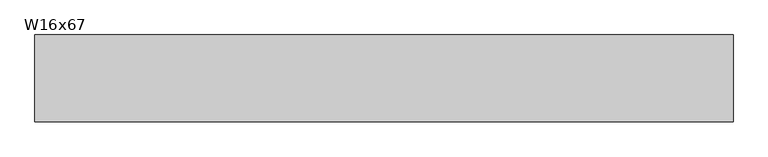
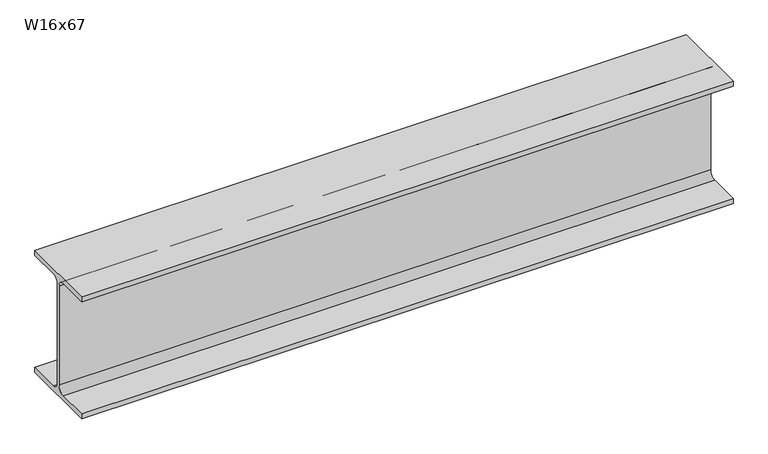
"""IFC4 building model written with IfcOpenShell, lengths in millimetres: beam geometry, RME W-Wide Flange : W16x67."""

from ifc_helpers import new_model, si_unit, point, frame, frame_2d, origin, place, context, project, spatial, polyline, circle_curve, trimmed, segment, composite_curve, outline, extrude, source, transform, mapped, element, save


def w16x67_bb9abaf4(model_context):
    return source(origin(), model_context, "Body", "SweptSolid", [
        extrude(outline(composite_curve([segment(polyline([(129.54, -190.119), (129.54, -207.01), (-129.54, -207.01), (-129.54, -190.119), (-27.813, -190.119)]), True, "CONTINUOUS"), segment(trimmed(circle_curve(frame_2d((-27.813, -167.3225)), 22.7965), [point((-27.813, -190.119))], [point((-5.0165, -167.3225))], True, "CARTESIAN"), True, "CONTINUOUS"), segment(polyline([(-5.0165, -167.3225), (-5.0165, 167.3225)]), True, "CONTINUOUS"), segment(trimmed(circle_curve(frame_2d((-27.813, 167.3225)), 22.7965), [point((-5.0165, 167.3225))], [point((-27.813, 190.119))], True, "CARTESIAN"), True, "CONTINUOUS"), segment(polyline([(-27.813, 190.119), (-129.54, 190.119), (-129.54, 207.01), (129.54, 207.01), (129.54, 190.119), (27.813, 190.119)]), True, "CONTINUOUS"), segment(trimmed(circle_curve(frame_2d((27.813, 167.3225)), 22.7965), [point((27.813, 190.119))], [point((5.0165, 167.3225))], True, "CARTESIAN"), True, "CONTINUOUS"), segment(polyline([(5.0165, 167.3225), (5.0165, -167.3225)]), True, "CONTINUOUS"), segment(trimmed(circle_curve(frame_2d((27.813, -167.3225)), 22.7965), [point((5.0165, -167.3225))], [point((27.813, -190.119))], True, "CARTESIAN"), True, "CONTINUOUS"), segment(polyline([(27.813, -190.119), (129.54, -190.119)]), True, "CONTINUOUS")], self_intersect=False)), frame((-906.4610687, 0.0, 0.0), z_axis=(1.0, 0.0, 0.0), x_axis=(0.0, 1.0, 0.0)), (0.0, 0.0, 1.0), 2085.9721374),
    ])


if __name__ == "__main__":
    model = new_model("IFC4")
    model_context = context("Model", 3, world=origin())
    ifc_project = project(units=[si_unit("LENGTHUNIT", "METRE", prefix="MILLI")], contexts=[model_context])
    site = spatial("IfcSite", under=ifc_project)
    building = spatial("IfcBuilding", under=site)
    placement = place(None, origin())
    w16x67_shape = w16x67_bb9abaf4(model_context)
    element("IfcBeam", 1, ObjectType="RME W-Wide Flange : W16x67", at=placement, inside=building, context=model_context, shape_type="MappedRepresentation", body=[
        mapped(w16x67_shape, transform((0.0, 0.0, 0.0), x_axis=(1.0, 0.0, 0.0), y_axis=(0.0, 1.0, 0.0), z_axis=(0.0, 0.0, 1.0))),
    ])
    save(model, "model.ifc")

# Revit data of these elements
# Type "RME W-Wide Flange : W16x67"
#   WELD P [instance default] = ""
#   WELD LE [instance default] = ""
#   WELD D [instance default] = ""
#   TOP SECTION SIZE [instance default] = ""
#   TOP SECTION LENGTH [instance default] = ""
#   REMARKS [instance default] = ""
#   REINF TYPE [instance default] = ""
#   Nominal Size = "W24"
#   End Bearing Capacity [instance default] = ""
#   BOT SECTION SIZE [instance default] = ""
#   BOT SECTION LENGTH [instance default] = ""
#   Assembly Code = "B10"
#   W = 67
#   Start Extension Calculation [instance default] = 10' - 0"
#   Start Extension [instance default] = -0' - 0 1/2"
#   End Extension Calculation [instance default] = 10' - 0"
#   End Extension [instance default] = -0' - 0 1/2"
#   Length [instance default] = 5' - 0"
#   bf = 0' - 10.2"
#   d = 1' - 4.3"
#   k = 0' - 1 9/16"
#   k2 = 0' - 0.8975"
#   tf = 0' - 0.665"
#   tw = 0' - 0.395"
#   A = 0.136806 SF
#   Structural Material [instance default] = Metal - Steel - ASTM A992
# Element 1 (IfcBeam, "RME W-Wide Flange : W16x67")
#   End Extension Calculation = 10' - 6 3/4"
#   End Extension = 0' - 6 1/4"
#   Length = 6' - 7.37489"
#   Materials on its faces: "Metal - Steel - ASTM A992"
# Materials
#   "Metal - Steel - ASTM A992": class "Metal", colour RGB 255 128 0, transparency 0
